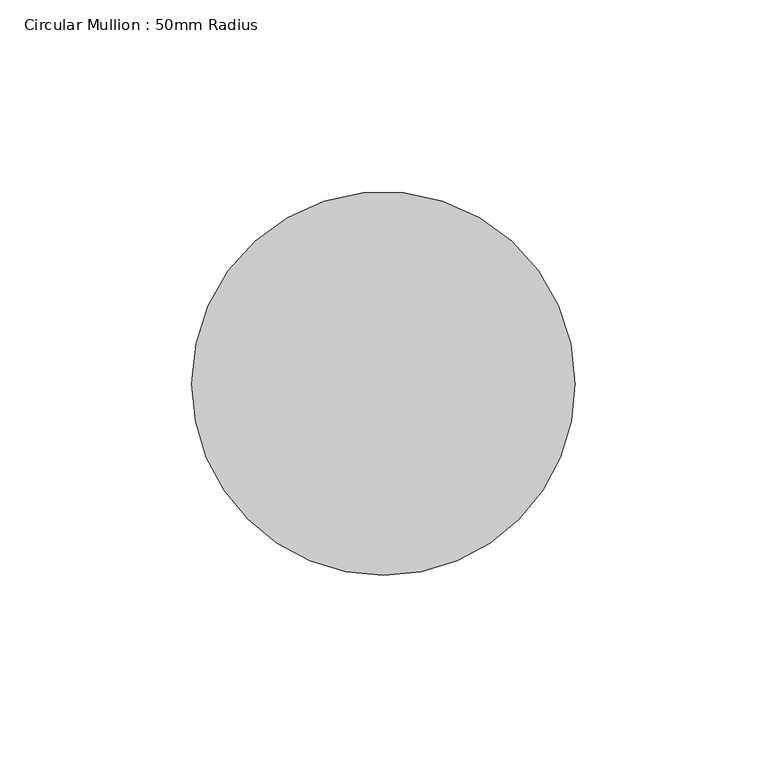
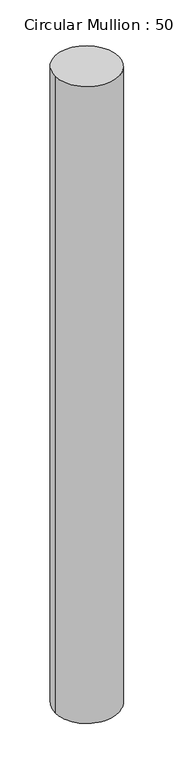
"""IFC4 building model written with IfcOpenShell, lengths in millimetres: member geometry, Circular Mullion : 50mm Radius."""

from ifc_helpers import new_model, si_unit, frame, origin, place, context, project, spatial, ellipse_curve, source, transform, mapped, element, save
from ifc_brep_helpers import plane_surface, cylinder_surface, advanced_brep


def circular_mullion_50mm_radius_9fc24fd1(model_context):
    return source(origin(), model_context, "Body", "AdvancedBrep", [
        advanced_brep(
        [(-100.0, 0.0, 1.3416911), (0.0, 0.0, 0.0), (0.0, 0.0, -1053.4886243), (-100.0, 0.0, -1054.8643489)],
        [
            (0, 1, ellipse_curve(frame((-50.0, 0.0, 0.6708456), z_axis=(-0.013414147970110328, -0.0152291831357633, -0.9997940450989162), x_axis=(-0.6608378922664468, -0.7502542320840944, 0.020294516124952793)), 50.0102999, 50.0)),
            (1, 2),
            (2, 3, ellipse_curve(frame((-50.0, 0.0, -1054.1764866), z_axis=(-0.013754267611395981, -0.01561532352401295, 0.9997834674536856), x_axis=(0.6608309007177108, 0.7502462945262272, 0.02080908951119287)), 50.010829, 50.0)),
            (3, 0),
            (1, 0, ellipse_curve(frame((-50.0, 0.0, 0.6708456), z_axis=(-0.013414147970110328, -0.0152291831357633, -0.9997940450989162), x_axis=(-0.6608378922664468, -0.7502542320840944, 0.020294516124952793)), 50.0102999, 50.0)),
            (3, 2, ellipse_curve(frame((-50.0, 0.0, -1054.1764866), z_axis=(-0.013754267611395981, -0.01561532352401295, 0.9997834674536856), x_axis=(0.6608309007177108, 0.7502462945262272, 0.02080908951119287)), 50.010829, 50.0)),
        ],
        [
            cylinder_surface(frame((-50.0, 0.0, 0.0), z_axis=(0.0, 0.0, 1.0), x_axis=(1.0, 0.0, 0.0)), 50.0),
            plane_surface(frame((-228.7245969, 201.4648822, 0.0), z_axis=(0.013414147970110328, 0.0152291831357633, 0.9997940450989162), x_axis=(0.6608378922664454, 0.7502542320840953, -0.020294516124969138))),
            plane_surface(frame((-228.7245969, 201.4648822, -1053.4886243), z_axis=(0.013754267611395978, 0.015615323524012946, -0.9997834674536854), x_axis=(0.6608309007177106, 0.7502462945262268, 0.020809089511208523))),
        ],
        [
            (0, [[1, 2, 3, 4]]),
            (0, [[5, -4, 6, -2]]),
            (1, [[-1, -5]]),
            (2, [[-6, -3]]),
        ],
    ),
    ])


if __name__ == "__main__":
    model = new_model("IFC4")
    model_context = context("Model", 3, world=origin())
    ifc_project = project(units=[si_unit("LENGTHUNIT", "METRE", prefix="MILLI")], contexts=[model_context])
    site = spatial("IfcSite", under=ifc_project)
    building = spatial("IfcBuilding", under=site)
    placement = place(None, origin())
    circular_mullion_50mm_radius_shape = circular_mullion_50mm_radius_9fc24fd1(model_context)
    element("IfcMember", 1, ObjectType="Circular Mullion : 50mm Radius", at=placement, inside=building, context=model_context, shape_type="MappedRepresentation", body=[
        mapped(circular_mullion_50mm_radius_shape, transform((0.0, 0.0, 0.0), x_axis=(1.0, 0.0, 0.0), y_axis=(0.0, 1.0, 0.0), z_axis=(0.0, 0.0, 1.0))),
    ])
    save(model, "model.ifc")

# Revit data of these elements
# Type "Circular Mullion : 50mm Radius"
#   built-in parameter 1007350 = 0.164042 (stored number, unit not read)
# Element 1 (IfcMember, "Circular Mullion : 50mm Radius")
#   Materials on its faces: "Aluminium"
# Materials
#   "Aluminium": class "Metal", colour RGB 247 247 247, transparency 0, Description = "Aluminium 6061", Cost = 0
